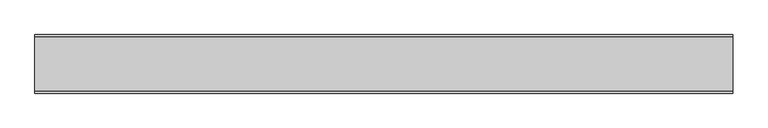
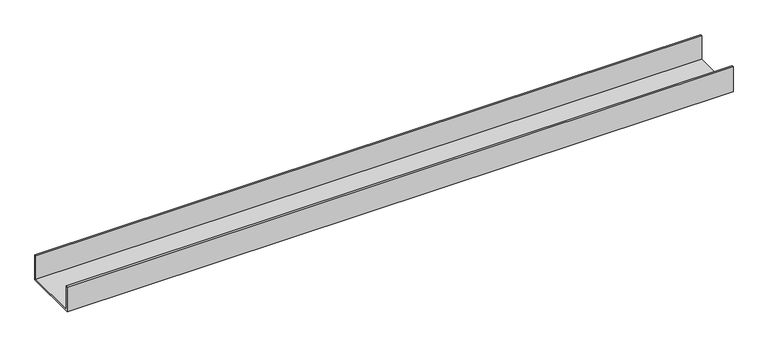
"""IFC4 building model written with IfcOpenShell, lengths in millimetres: proxy geometry, Generic Models 3:Generic Models 1:6:Generic Models 1:6 : Generic Models 3:Generic Models 1:300625:350611:Generic Models 1:6:Generic Models 1:6 : Generic Models 3:Generic Models 1:300625:350611 : Generic Models 3:Generic Models 1:6:Generic Models 1:6 : Generic Models 3:Generic Models 1:300625:350611:8 : Generic Models 3:Generic Models 1:6:Generic Models 1:6 : Generic Models 3:Generic Models 1:300625:350611:Generic Models 1:6:Generic Models 1:6 : Generic Models 3:Generic Models 1:300625:350611 : Generic Models 3:Generic Models 1:6:Generic Models 1:6 : Generic Models 3:Generic Models 1:300625:350611:301824."""

from ifc_helpers import new_model, si_unit, frame, origin, place, context, project, spatial, polyline, outline, extrude, source, transform, mapped, element, save


def generic_models_e61460fe(model_context):
    return source(origin(), model_context, "Body", "SweptSolid", [
        extrude(outline(polyline([(-578797.4913841, 0.0), (-579000.6913841, 0.0), (-579000.6913841, 95.25), (-578994.3413841, 95.25), (-578994.3413841, 6.35), (-578803.8413841, 6.35), (-578803.8413841, 95.25), (-578797.4913841, 95.25), (-578797.4913841, 0.0)])), frame((593757.1367239, 0.0, 0.0), z_axis=(1.0, 0.0, 0.0), x_axis=(0.0, 1.0, 0.0)), (0.0, 0.0, 1.0), 2419.35),
    ])


if __name__ == "__main__":
    model = new_model("IFC4")
    model_context = context("Model", 3, world=origin())
    ifc_project = project(units=[si_unit("LENGTHUNIT", "METRE", prefix="MILLI")], contexts=[model_context])
    site = spatial("IfcSite", under=ifc_project)
    building = spatial("IfcBuilding", under=site)
    placement = place(None, origin())
    generic_models_shape = generic_models_e61460fe(model_context)
    element("IfcBuildingElementProxy", 1, Name="Generic Models 3:Generic Models 1:6:Generic Models 1:6 : Generic Models 3:Generic Models 1:300625:350611:Generic Models 1:6:Generic Models 1:6 : Generic Models 3:Generic Models 1:300625:350611 : Generic Models 3:Generic Models 1:6:Generic Models 1:6 : Generic Models 3:Generic Models 1:300625:350611:8 : Generic Models 3:Generic Models 1:6:Generic Models 1:6 : Generic Models 3:Generic Models 1:300625:350611:Generic Models 1:6:Generic Models 1:6 : Generic Models 3:Generic Models 1:300625:350611 : Generic Models 3:Generic Models 1:6:Generic Models 1:6 : Generic Models 3:Generic Models 1:300625:350611:301824", ObjectType="Generic Models 3:Generic Models 1:6:Generic Models 1:6 : Generic Models 3:Generic Models 1:300625:350611:Generic Models 1:6:Generic Models 1:6 : Generic Models 3:Generic Models 1:300625:350611 : Generic Models 3:Generic Models 1:6:Generic Models 1:6 : Generic Models 3:Generic Models 1:300625:350611:8 : Generic Models 3:Generic Models 1:6:Generic Models 1:6 : Generic Models 3:Generic Models 1:300625:350611:Generic Models 1:6:Generic Models 1:6 : Generic Models 3:Generic Models 1:300625:350611 : Generic Models 3:Generic Models 1:6:Generic Models 1:6 : Generic Models 3:Generic Models 1:300625:350611:301824", at=placement, inside=building, context=model_context, shape_type="MappedRepresentation", body=[
        mapped(generic_models_shape, transform((0.0, 0.0, 0.0), x_axis=(1.0, 0.0, 0.0), y_axis=(0.0, 1.0, 0.0), z_axis=(0.0, 0.0, 1.0))),
    ])
    save(model, "model.ifc")

# Revit data of these elements
# Type "Generic Models 3:Generic Models 1:6:Generic Models 1:6 : Generic Models 3:Generic Models 1:300625:350611:Generic Models 1:6:Generic Models 1:6 : Generic Models 3:Generic Models 1:300625:350611 : Generic Models 3:Generic Models 1:6:Generic Models 1:6 : Generic Models 3:Generic Models 1:300625:350611:8 : Generic Models 3:Generic Models 1:6:Generic Models 1:6 : Generic Models 3:Generic Models 1:300625:350611:Generic Models 1:6:Generic Models 1:6 : Generic Models 3:Generic Models 1:300625:350611 : Generic Models 3:Generic Models 1:6:Generic Models 1:6 : Generic Models 3:Generic Models 1:300625:350611:301824"
#   NameOverride = "Generic Models 3:Generic Models 1:6:Generic Models 1:6 : Generic Models 3:Generic Models 1:300625:350611:Generic Models 1:6:Generic Models 1:6 : Generic Models 3:Generic Models 1:300625:350611 : Generic Models 3:Generic Models 1:6:Generic Models 1:6 : Generic Models 3:Generic Models 1:300625:350611:301824"
#   ObjectTypeOverride = "Generic Models 1:6:Generic Models 1:6 : Generic Models 3:Generic Models 1:300625:350611 : Generic Models 3:Generic Models 1:6:Generic Models 1:6 : Generic Models 3:Generic Models 1:300625:350611"
#   Reference = "Generic Models 1"
#   Tag = "301824"
